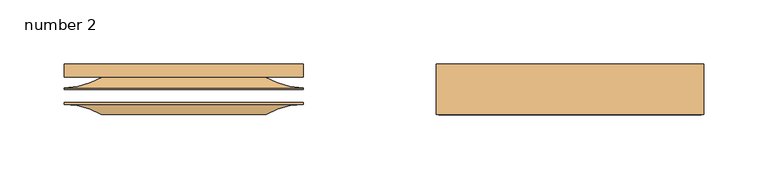
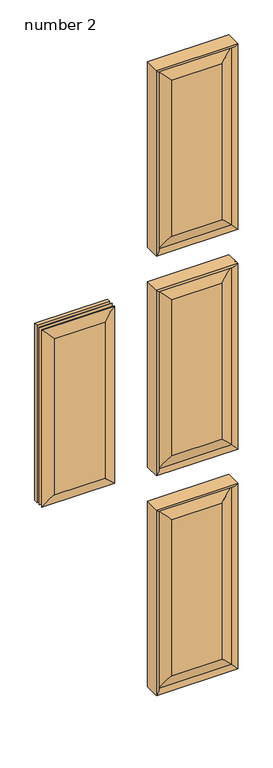
# IFC4 building model written with IfcOpenShell, lengths in millimetres: door geometry, Door-Interior-Karona-K5660-6_Panel : number 2.
# Revit data of these elements (continued)
# Type "Door-Interior-Karona-K5660-6_Panel : number 2" (continued)
#   Daylight Opening Width = 0' - 0"
#   Daylight Opening Height = 0' - 0"
#   Bottom Rail Height = 0' - 8 1/2"
#   3D Open Angle = 0.00°
#   Thickness = 0' - 1 3/4"
#   Stop Thickness = 0' - 0 1/2"
#   Stop Depth = 0' - 1 3/8"
#   Rough Width = 2' - 7 29/32"
#   Rough Height = 6' - 8 61/64"
#   Rabbet Width = 0' - 1 3/4"
#   Jamb Offset = 0' - 0 61/64"
#   Hinge Offset = 0' - 0 3/4"
#   Jamb Thickness = 0' - 0 29/32"
#   Ext. Frame Thickness = 0' - 0 5/8"
#   Int. Frame Thickness = 0' - 0 5/8"
#   Height = 6' - 8"
#   Width = 2' - 6"
#   3D Angle = 0.00°
#   Trim Visible = yes
#   Square Sticking Profile = no
#   Raised Panel Door = yes
#   Ovolo Sticking Profile = yes
#   Ogee Sticking Profile = no
#   Mission Sticking Profile = no
#   Hinge Visible = yes
#   Glass Panel Door = no
#   Flat Panel Door = no
#   Edition number = 1
#   Define Thermal Properties by = 1
#   Trim Material = Wood - Karona - Red Oak
#   Top Rail Material = Wood - Karona - Red Oak
#   Stile Material = Wood - Karona - Red Oak
#   Sticking Material = Wood - Karona - Red Oak
#   Jamb Material = Wood - Karona - Red Oak
#   Interior Panel = Wood - Karona - Red Oak
#   Door Panel Material = Wood - Karona - Red Oak
#   Bottom Rail Material = Wood - Karona - Red Oak
#   Visual Light Transmittance = 0
#   Solar Heat Gain Coefficient = 0
#   Construction Type = (empty or 0)
#   Function = (empty or 0)
#   Wall Closure = (empty or 0)
# Element 1 (IfcDoor, "Door-Interior-Karona-K5660-6_Panel : number 2")
#   Materials on its faces: "Wood - Karona - Red Oak"
# Materials
#   "Wood - Karona - Red Oak": class "Wood", colour RGB 153 121 89, transparency 0, Description = "Quercus Rubra", Cost = 0
